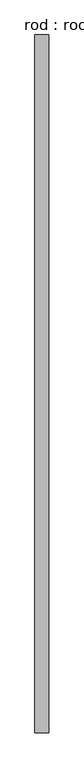
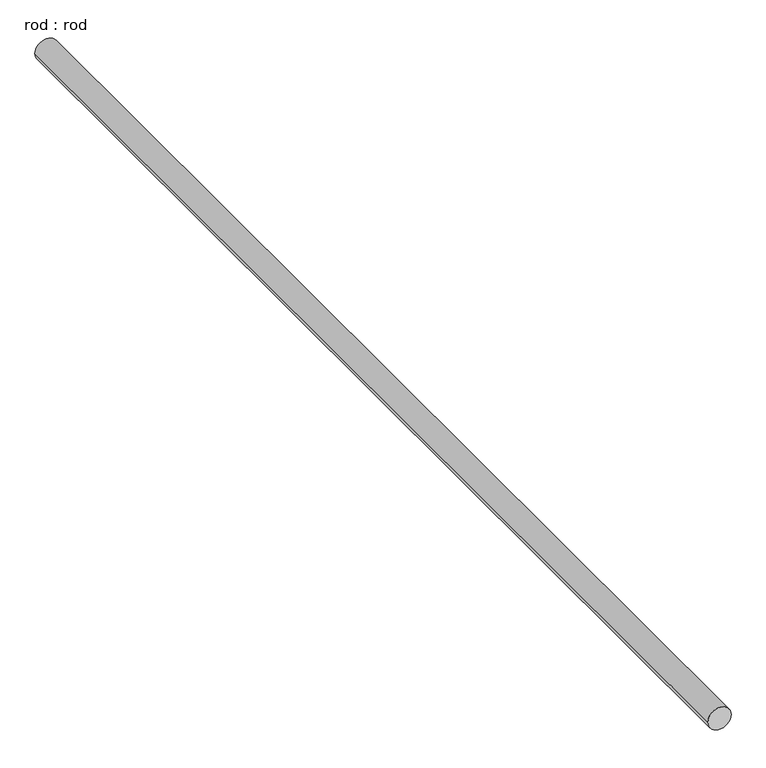
"""IFC4 building model written with IfcOpenShell, lengths in millimetres: proxy geometry, rod : rod."""

from ifc_helpers import new_model, si_unit, point, frame, frame_2d, origin, place, context, project, spatial, circle_curve, trimmed, segment, composite_curve, outline, extrude, source, transform, mapped, element, save


def rod_rod_aca0a701(model_context):
    return source(origin(), model_context, "Body", "SweptSolid", [
        extrude(outline(composite_curve([segment(trimmed(circle_curve(frame_2d((0.0108462, 0.0)), 200.0), [point((0.0108462, 200.0))], [point((0.0108462, -200.0))], False, "CARTESIAN"), True, "CONTINUOUS"), segment(trimmed(circle_curve(frame_2d((0.0108462, 0.0)), 200.0), [point((0.0108462, -200.0))], [point((0.0108462, 200.0))], False, "CARTESIAN"), True, "CONTINUOUS")], self_intersect=False)), frame((0.0, -5980.2165948, 0.0), z_axis=(0.0, 1.0, 0.0), x_axis=(0.0, 0.0, 1.0)), (0.0, 0.0, 1.0), 20145.8904203),
    ])


if __name__ == "__main__":
    model = new_model("IFC4")
    model_context = context("Model", 3, world=origin())
    ifc_project = project(units=[si_unit("LENGTHUNIT", "METRE", prefix="MILLI")], contexts=[model_context])
    site = spatial("IfcSite", under=ifc_project)
    building = spatial("IfcBuilding", under=site)
    placement = place(None, origin())
    rod_rod_shape = rod_rod_aca0a701(model_context)
    element("IfcBuildingElementProxy", 1, Name="rod : rod", ObjectType="rod : rod", at=placement, inside=building, context=model_context, shape_type="MappedRepresentation", body=[
        mapped(rod_rod_shape, transform((0.0, 0.0, 0.0), x_axis=(1.0, 0.0, 0.0), y_axis=(0.0, 1.0, 0.0), z_axis=(0.0, 0.0, 1.0))),
    ])
    save(model, "model.ifc")

# Revit data of these elements
# Type "rod : rod"
#   Default Elevation = 0
